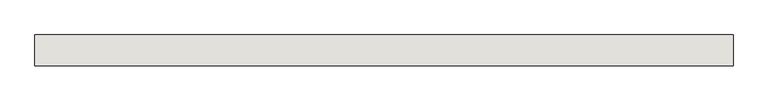
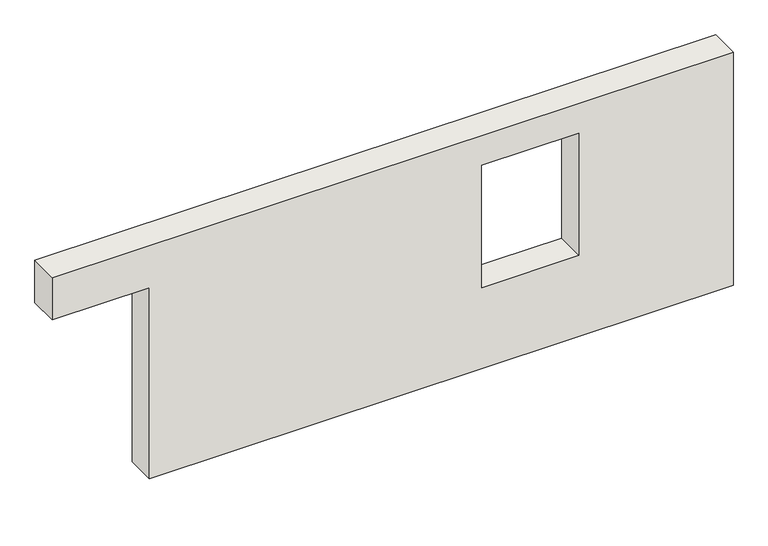
"""IFC4 building model written with IfcOpenShell, lengths in millimetres: wall geometry, 0_3d_modell."""

from ifc_helpers import new_model, si_unit, frame, origin, place, context, project, spatial, polyline, outline, extrude, source, transform, mapped, element, save


def wall_8b87bf5e(model_context):
    return source(origin(), model_context, "Body", "SweptSolid", [
        extrude(outline(polyline([(2360.0, 0.0), (2360.0, 1135.0), (0.0, 1135.0), (0.0, 7950.0), (2880.0, 7950.0), (2880.0, 0.0), (2360.0, 0.0)]), holes=[polyline([(1000.0, 5015.0), (2510.0, 5015.0), (2510.0, 6150.0), (1000.0, 6150.0), (1000.0, 5015.0)])]), frame((0.0, 0.0, 0.0), z_axis=(0.0, 1.0, 0.0), x_axis=(0.0, 0.0, 1.0)), (0.0, 0.0, 1.0), 350.0),
    ])


if __name__ == "__main__":
    model = new_model("IFC4")
    model_context = context("Model", 3, world=origin())
    ifc_project = project(units=[si_unit("LENGTHUNIT", "METRE", prefix="MILLI")], contexts=[model_context])
    site = spatial("IfcSite", under=ifc_project)
    building = spatial("IfcBuilding", under=site)
    placement = place(None, origin())
    wall_shape = wall_8b87bf5e(model_context)
    element("IfcWall", 1, ObjectType="0_3d_modell", at=placement, inside=building, context=model_context, shape_type="MappedRepresentation", body=[
        mapped(wall_shape, transform((0.0, 0.0, 0.0), x_axis=(1.0, 0.0, 0.0), y_axis=(0.0, 1.0, 0.0), z_axis=(0.0, 0.0, 1.0))),
    ])
    save(model, "model.ifc")

# Revit data of these elements
# Element 1 (IfcWall, "0_3d_modell")
#   Materials on its faces: "holzschalung"
# Materials
#   "holzschalung": class "Unassigned", colour RGB 128 128 128, transparency 0
